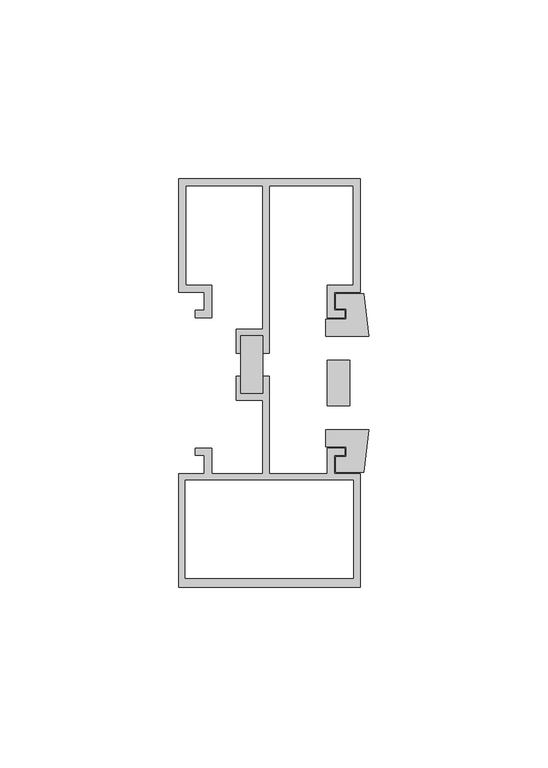
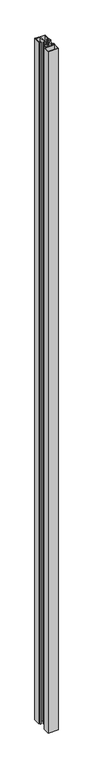
"""IFC4 building model written with IfcOpenShell, lengths in millimetres: proxy geometry, Generic Models 3:Generic Models 1:5:Generic Models 1:5 : Generic Models 3:Generic Models 1:300625:345888:Generic Models 1:5:Generic Models 1:5 : Generic Models 3:Generic Models 1:300625:345888 : Generic Models 3:Generic Models 1:5:Generic Models 1:5 : Generic Models 3:Generic Models 1:300625:345888:3 : Generic Models 3:Generic Models 1:5:Generic Models 1:5 : Generic Models 3:Generic Models 1:300625:345888:Generic Models 1:5:Generic Models 1:5 : Generic Models 3:Generic Models 1:300625:345888 : Generic Models 3:Generic Models 1:5:Generic Models 1:5 : Generic Models 3:Generic Models 1:300625:345888:301574."""

from ifc_helpers import new_model, si_unit, frame, origin, place, context, project, spatial, polyline, outline, extrude, source, transform, mapped, element, save


def generic_models_b8ffe188(model_context):
    return source(origin(), model_context, "Body", "SweptSolid", [
        extrude(outline(polyline([(569499.8074021, -579063.9802804), (569493.7276149, -579063.9802804), (569493.7276149, -579047.8688442), (569499.8074021, -579047.8688442), (569499.8074021, -579063.9802804)])), frame((0.0, 0.0, 66.3122056), z_axis=(0.0, 0.0, 1.0), x_axis=(1.0, 0.0, 0.0)), (0.0, 0.0, 1.0), 3584.971571),
        extrude(outline(polyline([(569524.2383176, -579067.3663841), (569517.8947692, -579067.3663841), (569517.8947692, -579054.6663841), (569524.2383176, -579054.6663841), (569524.2383176, -579067.3663841)])), frame((0.0, 0.0, 66.3122056), z_axis=(0.0, 0.0, 1.0), x_axis=(1.0, 0.0, 0.0)), (0.0, 0.0, 1.0), 3584.971571),
        extrude(outline(polyline([(569523.2114348, -579078.8588708), (569517.4978941, -579078.8588708), (569517.4978941, -579074.1048149), (569529.5681513, -579074.1048149), (569528.1072844, -579086.0026208), (569520.267575, -579086.0026208), (569520.267575, -579081.704549), (569523.2114348, -579081.704549), (569523.2114348, -579078.8588708)])), frame((0.0, 0.0, 66.3122056), z_axis=(0.0, 0.0, 1.0), x_axis=(1.0, 0.0, 0.0)), (0.0, 0.0, 1.0), 3584.971571),
        extrude(outline(polyline([(569528.1072844, -579036.0301474), (569529.5681513, -579047.9279532), (569517.4978941, -579047.9279532), (569517.4978941, -579043.1738974), (569523.2114348, -579043.1738974), (569523.2114348, -579040.3282192), (569520.267575, -579040.3282192), (569520.267575, -579036.0301474), (569528.1072844, -579036.0301474)])), frame((0.0, 0.0, 66.3122056), z_axis=(0.0, 0.0, 1.0), x_axis=(1.0, 0.0, 0.0)), (0.0, 0.0, 1.0), 3584.9377944),
        extrude(outline(polyline([(569476.3242239, -579118.1663841), (569476.3242239, -579086.3994958), (569483.5439713, -579086.3994958), (569483.5439713, -579081.307674), (569481.0247398, -579081.307674), (569481.0247398, -579079.2557458), (569485.5958995, -579079.2557458), (569485.5958995, -579086.3994958), (569499.8074021, -579086.3994958), (569499.8074021, -579065.8802139), (569492.4356601, -579065.8802139), (569492.4356601, -579059.1164506), (569493.7276149, -579059.1164506), (569493.7276149, -579063.9802804), (569499.8074021, -579063.9802804), (569499.8074021, -579059.1164506), (569501.7073356, -579059.1164506), (569501.7073356, -579086.3994958), (569517.8947691, -579086.3994958), (569517.8947691, -579079.2557458), (569522.8145598, -579079.2557458), (569522.8145598, -579081.307674), (569519.8707, -579081.307674), (569519.8707, -579086.3994958), (569527.0904473, -579086.3994958), (569527.0904473, -579118.1663841), (569476.3242239, -579118.1663841)]), holes=[polyline([(569525.1905138, -579088.2994293), (569478.2241574, -579088.2994293), (569478.2241574, -579115.6584719), (569525.1905138, -579115.6584719), (569525.1905138, -579088.2994293)])]), frame((0.0, 0.0, 66.3122056), z_axis=(0.0, 0.0, 1.0), x_axis=(1.0, 0.0, 0.0)), (0.0, 0.0, 1.0), 3584.971571),
        extrude(outline(polyline([(569522.8145598, -579040.7250942), (569522.8145598, -579042.7770224), (569517.8947691, -579042.7770224), (569517.8947691, -579033.7333389), (569525.1806483, -579033.7333389), (569525.1806483, -579005.8423149), (569501.7073356, -579005.8423149), (569501.7073356, -579052.732674), (569499.8074021, -579052.732674), (569499.8074021, -579047.8688442), (569493.7276149, -579047.8688442), (569493.7276149, -579052.732674), (569492.4356601, -579052.732674), (569492.4356601, -579045.9689107), (569499.8074021, -579045.9689107), (569499.8074021, -579005.8423149), (569478.2464365, -579005.8423149), (569478.2464365, -579033.7333389), (569485.5958995, -579033.7333389), (569485.5958995, -579042.7770224), (569481.0247398, -579042.7770224), (569481.0247398, -579040.7250942), (569483.5439713, -579040.7250942), (569483.5439713, -579035.6332724), (569476.3242239, -579035.6332724), (569476.3242239, -579003.8663841), (569527.0904473, -579003.8663841), (569527.0904473, -579035.6332724), (569519.8707, -579035.6332724), (569519.8707, -579040.7250942), (569522.8145598, -579040.7250942)])), frame((0.0, 0.0, 66.3122056), z_axis=(0.0, 0.0, 1.0), x_axis=(1.0, 0.0, 0.0)), (0.0, 0.0, 1.0), 3584.971571),
    ])


if __name__ == "__main__":
    model = new_model("IFC4")
    model_context = context("Model", 3, world=origin())
    ifc_project = project(units=[si_unit("LENGTHUNIT", "METRE", prefix="MILLI")], contexts=[model_context])
    site = spatial("IfcSite", under=ifc_project)
    building = spatial("IfcBuilding", under=site)
    placement = place(None, origin())
    generic_models_shape = generic_models_b8ffe188(model_context)
    element("IfcBuildingElementProxy", 1, Name="Generic Models 3:Generic Models 1:5:Generic Models 1:5 : Generic Models 3:Generic Models 1:300625:345888:Generic Models 1:5:Generic Models 1:5 : Generic Models 3:Generic Models 1:300625:345888 : Generic Models 3:Generic Models 1:5:Generic Models 1:5 : Generic Models 3:Generic Models 1:300625:345888:3 : Generic Models 3:Generic Models 1:5:Generic Models 1:5 : Generic Models 3:Generic Models 1:300625:345888:Generic Models 1:5:Generic Models 1:5 : Generic Models 3:Generic Models 1:300625:345888 : Generic Models 3:Generic Models 1:5:Generic Models 1:5 : Generic Models 3:Generic Models 1:300625:345888:301574", ObjectType="Generic Models 3:Generic Models 1:5:Generic Models 1:5 : Generic Models 3:Generic Models 1:300625:345888:Generic Models 1:5:Generic Models 1:5 : Generic Models 3:Generic Models 1:300625:345888 : Generic Models 3:Generic Models 1:5:Generic Models 1:5 : Generic Models 3:Generic Models 1:300625:345888:3 : Generic Models 3:Generic Models 1:5:Generic Models 1:5 : Generic Models 3:Generic Models 1:300625:345888:Generic Models 1:5:Generic Models 1:5 : Generic Models 3:Generic Models 1:300625:345888 : Generic Models 3:Generic Models 1:5:Generic Models 1:5 : Generic Models 3:Generic Models 1:300625:345888:301574", at=placement, inside=building, context=model_context, shape_type="MappedRepresentation", body=[
        mapped(generic_models_shape, transform((0.0, 0.0, 0.0), x_axis=(1.0, 0.0, 0.0), y_axis=(0.0, 1.0, 0.0), z_axis=(0.0, 0.0, 1.0))),
    ])
    save(model, "model.ifc")

# Revit data of these elements
# Type "Generic Models 3:Generic Models 1:5:Generic Models 1:5 : Generic Models 3:Generic Models 1:300625:345888:Generic Models 1:5:Generic Models 1:5 : Generic Models 3:Generic Models 1:300625:345888 : Generic Models 3:Generic Models 1:5:Generic Models 1:5 : Generic Models 3:Generic Models 1:300625:345888:3 : Generic Models 3:Generic Models 1:5:Generic Models 1:5 : Generic Models 3:Generic Models 1:300625:345888:Generic Models 1:5:Generic Models 1:5 : Generic Models 3:Generic Models 1:300625:345888 : Generic Models 3:Generic Models 1:5:Generic Models 1:5 : Generic Models 3:Generic Models 1:300625:345888:301574"
#   NameOverride = "Generic Models 3:Generic Models 1:5:Generic Models 1:5 : Generic Models 3:Generic Models 1:300625:345888:Generic Models 1:5:Generic Models 1:5 : Generic Models 3:Generic Models 1:300625:345888 : Generic Models 3:Generic Models 1:5:Generic Models 1:5 : Generic Models 3:Generic Models 1:300625:345888:301574"
#   ObjectTypeOverride = "Generic Models 1:5:Generic Models 1:5 : Generic Models 3:Generic Models 1:300625:345888 : Generic Models 3:Generic Models 1:5:Generic Models 1:5 : Generic Models 3:Generic Models 1:300625:345888"
#   Reference = "Generic Models 1"
#   Tag = "301574"
# Element 1 (IfcBuildingElementProxy, "Generic Models 3:Generic Models 1:5:Generic Models 1:5 : Generic Models 3:Generic Models 1:300625:345888:Generic Models 1:5:Generic Models 1:5 : Generic Models 3:Generic Models 1:300625:345888 : Generic Models 3:Generic Models 1:5:Generic Models 1:5 : Generic Models 3:Generic Models 1:300625:345888:3 : Generic Models 3:Generic Models 1:5:Generic Models 1:5 : Generic Models 3:Generic Models 1:300625:345888:Generic Models 1:5:Generic Models 1:5 : Generic Models 3:Generic Models 1:300625:345888 : Generic Models 3:Generic Models 1:5:Generic Models 1:5 : Generic Models 3:Generic Models 1:300625:345888:301574")
#   Materials on its faces: "THERMAL BROKEN ALUMINUM STOREFRONT"
# Materials
#   "THERMAL BROKEN ALUMINUM STOREFRONT": class "Unassigned", colour RGB 244 244 244, transparency 0, Cost = 0
